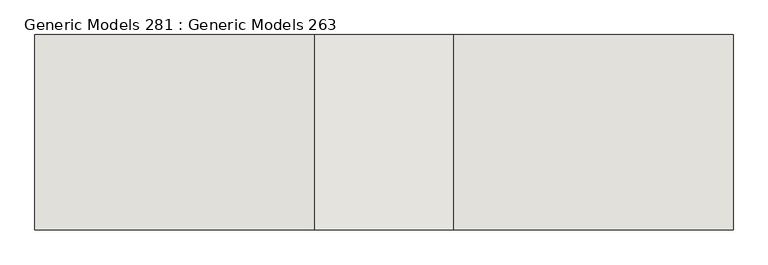
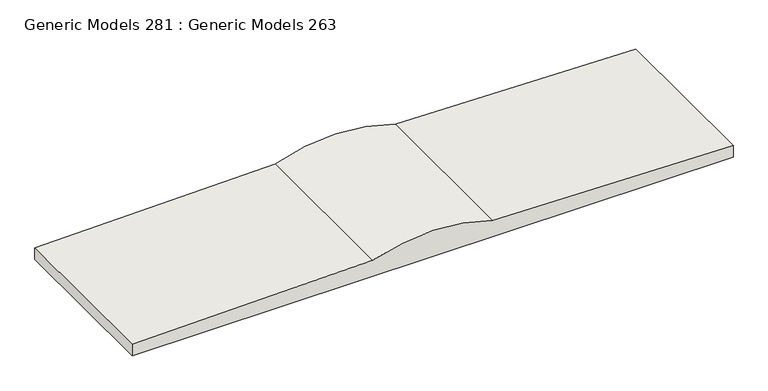
"""IFC4 building model written with IfcOpenShell, lengths in millimetres: wall geometry, Generic Models 281 : Generic Models 263."""

from ifc_helpers import new_model, si_unit, point, frame, frame_2d, origin, place, context, project, spatial, polyline, circle_curve, trimmed, segment, composite_curve, outline, extrude, source, transform, mapped, element, save


def generic_models_281_generic_models_263_cbb34a41(model_context):
    return source(origin(), model_context, "Body", "SweptSolid", [
        extrude(outline(composite_curve([segment(polyline([(0.0, 64122.5797726), (-304.9836851, 64122.5797726)]), True, "CONTINUOUS"), segment(trimmed(circle_curve(frame_2d((-219607.3320282, 71742.5797726)), 219434.6927648), [point((-304.9836851, 64122.5797726))], [point((-304.9836851, 79362.5797726))], True, "CARTESIAN"), True, "CONTINUOUS"), segment(polyline([(-304.9836851, 79362.5797726), (0.0, 79362.5797726)]), True, "CONTINUOUS"), segment(trimmed(circle_curve(frame_2d((-219607.3320282, 71742.5797726)), 219739.4927648), [point((0.0, 79362.5797726))], [point((126.8758334, 73266.5797726))], False, "CARTESIAN"), True, "CONTINUOUS"), segment(trimmed(circle_curve(frame_2d((-4163.1944851, 71742.5797726)), 4552.7221898), [point((126.8758334, 73266.5797726))], [point((126.8758334, 70218.5797726))], False, "CARTESIAN"), True, "CONTINUOUS"), segment(trimmed(circle_curve(frame_2d((-219607.3320282, 71742.5797726)), 219739.4927648), [point((126.8758334, 70218.5797726))], [point((0.0, 64122.5797726))], False, "CARTESIAN"), True, "CONTINUOUS")], self_intersect=False)), frame((0.0, -1618.4486541, 0.0), z_axis=(0.0, 1.0, 0.0), x_axis=(0.0, 0.0, 1.0)), (0.0, 0.0, 1.0), 4267.2),
    ])


if __name__ == "__main__":
    model = new_model("IFC4")
    model_context = context("Model", 3, world=origin())
    ifc_project = project(units=[si_unit("LENGTHUNIT", "METRE", prefix="MILLI")], contexts=[model_context])
    site = spatial("IfcSite", under=ifc_project)
    building = spatial("IfcBuilding", under=site)
    placement = place(None, origin())
    generic_models_281_generic_models_263_shape = generic_models_281_generic_models_263_cbb34a41(model_context)
    element("IfcWall", 1, ObjectType="Generic Models 281 : Generic Models 263", at=placement, inside=building, context=model_context, shape_type="MappedRepresentation", body=[
        mapped(generic_models_281_generic_models_263_shape, transform((0.0, 0.0, 0.0), x_axis=(1.0, 0.0, 0.0), y_axis=(0.0, 1.0, 0.0), z_axis=(0.0, 0.0, 1.0))),
    ])
    save(model, "model.ifc")

# Revit data of these elements
# Element 1 (IfcWall, "Generic Models 281 : Generic Models 263")
#   Materials on its faces: "3\" TO 6\" WASHED OR CLEAR STONE"
# Materials
#   "3\" TO 6\" WASHED OR CLEAR STONE": class "Miscellaneous", colour RGB 210 210 210, transparency 0, Cost = 0
